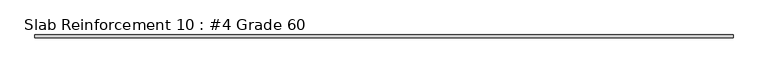
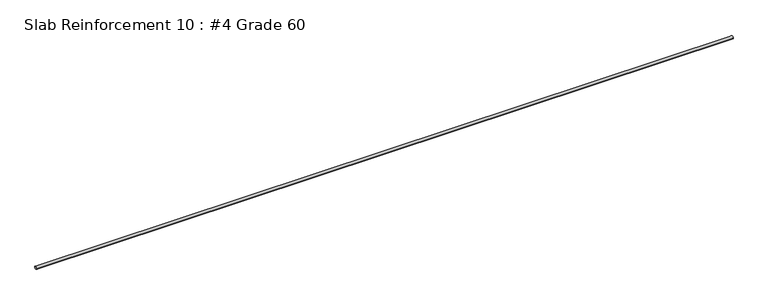
"""IFC4 building model written with IfcOpenShell, lengths in millimetres: proxy geometry, Slab Reinforcement 10 : #4 Grade 60."""

from ifc_helpers import new_model, si_unit, point, frame, frame_2d, origin, place, context, project, spatial, circle_curve, trimmed, segment, composite_curve, outline, extrude, source, transform, mapped, element, save


def slab_reinforcement_10_4_grade_60_863f9fcf(model_context):
    return source(origin(), model_context, "Body", "SweptSolid", [
        extrude(outline(composite_curve([segment(trimmed(circle_curve(frame_2d((-534045.8663841, -82.55)), 6.35), [point((-534052.2163841, -82.55))], [point((-534039.5163841, -82.55))], False, "CARTESIAN"), True, "CONTINUOUS"), segment(trimmed(circle_curve(frame_2d((-534045.8663841, -82.55)), 6.35), [point((-534039.5163841, -82.55))], [point((-534052.2163841, -82.55))], False, "CARTESIAN"), True, "CONTINUOUS")], self_intersect=False)), frame((587369.3484865, 0.0, 0.0), z_axis=(1.0, 0.0, 0.0), x_axis=(0.0, 1.0, 0.0)), (0.0, 0.0, 1.0), 2946.4),
    ])


if __name__ == "__main__":
    model = new_model("IFC4")
    model_context = context("Model", 3, world=origin())
    ifc_project = project(units=[si_unit("LENGTHUNIT", "METRE", prefix="MILLI")], contexts=[model_context])
    site = spatial("IfcSite", under=ifc_project)
    building = spatial("IfcBuilding", under=site)
    placement = place(None, origin())
    slab_reinforcement_10_4_grade_60_shape = slab_reinforcement_10_4_grade_60_863f9fcf(model_context)
    element("IfcBuildingElementProxy", 1, Name="Slab Reinforcement 10 : #4 Grade 60", ObjectType="Slab Reinforcement 10 : #4 Grade 60", at=placement, inside=building, context=model_context, shape_type="MappedRepresentation", body=[
        mapped(slab_reinforcement_10_4_grade_60_shape, transform((0.0, 0.0, 0.0), x_axis=(1.0, 0.0, 0.0), y_axis=(0.0, 1.0, 0.0), z_axis=(0.0, 0.0, 1.0))),
    ])
    save(model, "model.ifc")

# Revit data of these elements
# Element 1 (IfcBuildingElementProxy, "Slab Reinforcement 10 : #4 Grade 60")
#   Materials on its faces: "#4 GR. 60 REINF. @ 16\" O.C. EW."
# Materials
#   "#4 GR. 60 REINF. @ 16\" O.C. EW.": class "Generic", colour RGB 84 83 81, transparency 0, Cost = 0
